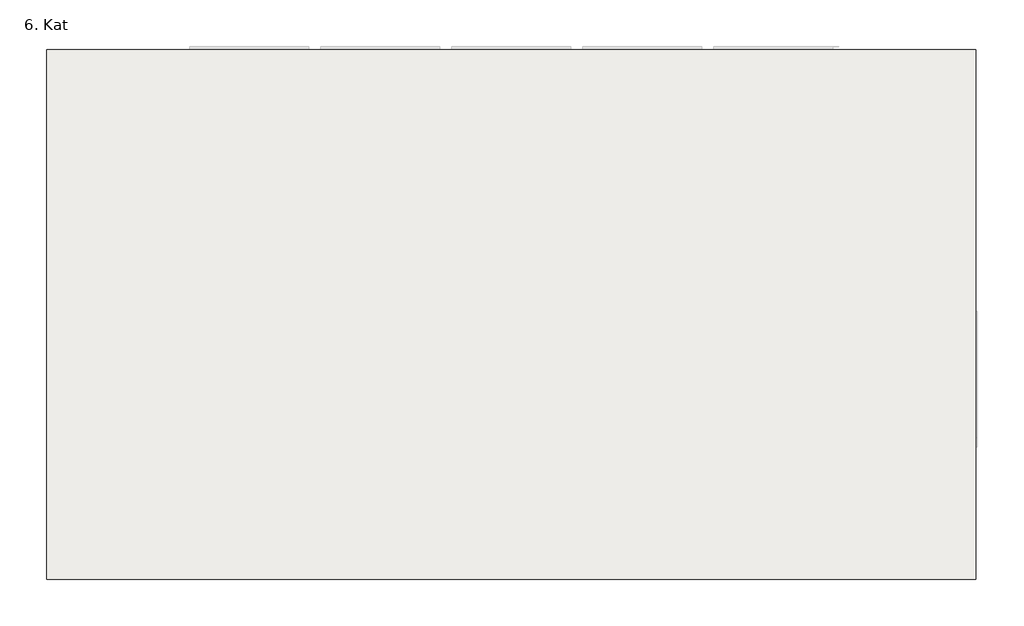
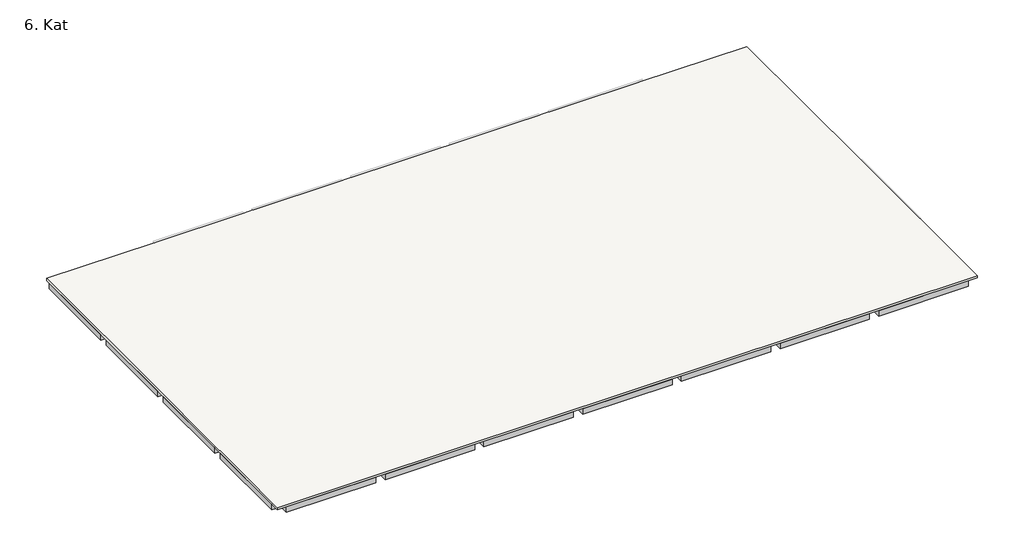
# One storey, part 1 of 2: 41 beams, 1 slab.
"""IFC4 building model written with IfcOpenShell, lengths in millimetres."""

from ifc_helpers import new_model, si_unit, frame, origin, place, context, project, spatial, polyline, outline, extrude, faceted_brep, element, save

model = new_model("IFC4")

# Units and contexts
model_context = context("Model", 3, world=origin())
ifc_project = project(units=[si_unit("LENGTHUNIT", "METRE", prefix="MILLI")], contexts=[model_context])

# Site, building, storey
site = spatial("IfcSite", under=ifc_project)
building = spatial("IfcBuilding", under=site)
storey = spatial("IfcBuildingStorey", under=building, Name="6. Kat", Elevation=31100.0)

# Beams
placement = place(None, origin())
element("IfcBeam", 1, ObjectType="M_Concrete-Rectangular Beam : 60x70cm kiriş", at=placement, inside=storey, context=model_context, shape_type="SweptSolid", body=[
    extrude(outline(polyline([(199.9996111, 8099.9999582), (199.9996111, 399.9999408), (-400.0003889, 399.9999408), (-400.0003889, 8099.9999582), (199.9996111, 8099.9999582)])), frame((0.0, 0.0, 30400.0), z_axis=(0.0, 0.0, 1.0), x_axis=(1.0, 0.0, 0.0)), (0.0, 0.0, 1.0), 500.0),
])
element("IfcBeam", 2, ObjectType="M_Concrete-Rectangular Beam : 60x70cm kiriş", at=placement, inside=storey, context=model_context, shape_type="SweptSolid", body=[
    extrude(outline(polyline([(199.9996411, 16599.9999423), (199.9996411, 8899.9999251), (-400.0003589, 8899.9999251), (-400.0003589, 16599.9999423), (199.9996411, 16599.9999423)])), frame((0.0, 0.0, 30400.0), z_axis=(0.0, 0.0, 1.0), x_axis=(1.0, 0.0, 0.0)), (0.0, 0.0, 1.0), 500.0),
])
element("IfcBeam", 3, ObjectType="M_Concrete-Rectangular Beam : 60x70cm kiriş", at=placement, inside=storey, context=model_context, shape_type="Brep", body=[
    faceted_brep([(199.9994072, 17399.9999423, 30400.0), (199.9994072, 23399.9999249, 30400.0), (199.9994072, 23899.9999249, 30400.0), (199.9994072, 25099.999926, 30400.0), (199.9994072, 25099.999926, 30900.0), (199.9994072, 23899.9999249, 30900.0), (199.9994072, 23399.9999249, 30900.0), (199.9994072, 17399.9999423, 30900.0), (-400.0005928, 17399.9999423, 30400.0), (-400.0005928, 25099.999926, 30400.0), (-400.0005928, 17399.9999423, 30900.0), (-400.0005928, 25099.999926, 30900.0)], [[[0, 1, 2, 3, 4, 5, 6, 7]], [[3, 2, 1, 0, 8, 9]], [[9, 8, 10, 11]], [[7, 6, 5, 4, 11, 10]], [[8, 0, 7, 10]], [[3, 9, 11, 4]]]),
])
element("IfcBeam", 4, ObjectType="M_Concrete-Rectangular Beam : 60x70cm kiriş", at=placement, inside=storey, context=model_context, shape_type="SweptSolid", body=[
    extrude(outline(polyline([(199.9994681, 25899.9999188), (-400.0005319, 25899.9999188), (-400.0005319, 33600.0004302), (199.9994681, 33600.0004302), (199.9994681, 25899.9999188)])), frame((0.0, 0.0, 30400.0), z_axis=(0.0, 0.0, 1.0), x_axis=(1.0, 0.0, 0.0)), (0.0, 0.0, 1.0), 500.0),
])
element("IfcBeam", 5, ObjectType="M_Concrete-Rectangular Beam : 60x70cm kiriş", at=placement, inside=storey, context=model_context, shape_type="SweptSolid", body=[
    extrude(outline(polyline([(8099.9996095, -400.0004808), (399.9996111, -400.0004808), (399.9996111, 199.9995192), (8099.9996095, 199.9995192), (8099.9996095, -400.0004808)])), frame((0.0, 0.0, 30400.0), z_axis=(0.0, 0.0, 1.0), x_axis=(1.0, 0.0, 0.0)), (0.0, 0.0, 1.0), 500.0),
])
element("IfcBeam", 6, ObjectType="M_Concrete-Rectangular Beam : 60x70cm kiriş", at=placement, inside=storey, context=model_context, shape_type="SweptSolid", body=[
    extrude(outline(polyline([(16599.9996095, -400.0000423), (8899.9996095, -400.0000423), (8899.9996095, 199.9999577), (16599.9996095, 199.9999577), (16599.9996095, -400.0000423)])), frame((0.0, 0.0, 30400.0), z_axis=(0.0, 0.0, 1.0), x_axis=(1.0, 0.0, 0.0)), (0.0, 0.0, 1.0), 500.0),
])
element("IfcBeam", 7, ObjectType="M_Concrete-Rectangular Beam : 60x70cm kiriş", at=placement, inside=storey, context=model_context, shape_type="SweptSolid", body=[
    extrude(outline(polyline([(25099.9996096, -399.9996163), (17399.9993907, -399.9996163), (17399.9993907, 200.0003837), (25099.9996096, 200.0003837), (25099.9996096, -399.9996163)])), frame((0.0, 0.0, 30400.0), z_axis=(0.0, 0.0, 1.0), x_axis=(1.0, 0.0, 0.0)), (0.0, 0.0, 1.0), 500.0),
])
element("IfcBeam", 8, ObjectType="M_Concrete-Rectangular Beam : 60x70cm kiriş", at=placement, inside=storey, context=model_context, shape_type="SweptSolid", body=[
    extrude(outline(polyline([(8899.9996095, 8100.0003637), (8899.9996095, 399.9999384), (8299.9996095, 399.9999384), (8299.9996095, 8100.0003637), (8899.9996095, 8100.0003637)])), frame((0.0, 0.0, 30400.0), z_axis=(0.0, 0.0, 1.0), x_axis=(1.0, 0.0, 0.0)), (0.0, 0.0, 1.0), 500.0),
])
element("IfcBeam", 9, ObjectType="M_Concrete-Rectangular Beam : 60x70cm kiriş", at=placement, inside=storey, context=model_context, shape_type="Brep", body=[
    faceted_brep([(8899.9996095, 8900.0003637, 30400.0), (8899.9996095, 13300.0003638, 30400.0), (8899.9996095, 13700.0003638, 30400.0), (8899.9996095, 16599.9999418, 30400.0), (8899.9996095, 16599.9999418, 30900.0), (8899.9996095, 13700.0003638, 30900.0), (8899.9996095, 13300.0003638, 30900.0), (8899.9996095, 8900.0003637, 30900.0), (8299.9996095, 8900.0003637, 30400.0), (8299.9996095, 16599.9999418, 30400.0), (8299.9996095, 8900.0003637, 30900.0), (8299.9996095, 16599.9999418, 30900.0)], [[[0, 1, 2, 3, 4, 5, 6, 7]], [[3, 2, 1, 0, 8, 9]], [[9, 8, 10, 11]], [[7, 6, 5, 4, 11, 10]], [[8, 0, 7, 10]], [[3, 9, 11, 4]]]),
])
element("IfcBeam", 10, ObjectType="M_Concrete-Rectangular Beam : 60x70cm kiriş", at=placement, inside=storey, context=model_context, shape_type="Brep", body=[
    faceted_brep([(8899.9996735, 25100.0003646, 30400.0), (8899.9996735, 25100.0003646, 30900.0), (8899.9996735, 17400.0009197, 30900.0), (8899.9996735, 17400.0009197, 30400.0), (8299.9996735, 25100.0003646, 30400.0), (8299.9996735, 17400.0009197, 30400.0), (8299.9996735, 18150.0006424, 30400.0), (8299.9996735, 18550.0006424, 30400.0), (8299.9996735, 23399.9999249, 30400.0), (8299.9996735, 23899.9999249, 30400.0), (8299.9996735, 25100.0003646, 30900.0), (8299.9996735, 17400.0009197, 30900.0), (8299.9996735, 18150.0006424, 30900.0), (8299.9996735, 18550.0006424, 30900.0), (8299.9996735, 23399.9999249, 30900.0), (8299.9996735, 23899.9999249, 30900.0)], [[[0, 1, 2, 3]], [[4, 0, 3, 5, 6, 7, 8, 9]], [[10, 4, 9, 8, 7, 6, 5, 11, 12, 13, 14, 15]], [[1, 10, 15, 14, 13, 12, 11, 2]], [[0, 4, 10, 1]], [[3, 2, 11, 5]]]),
])
element("IfcBeam", 11, ObjectType="M_Concrete-Rectangular Beam : 60x70cm kiriş", at=placement, inside=storey, context=model_context, shape_type="SweptSolid", body=[
    extrude(outline(polyline([(8899.9993907, 25899.9999188), (8299.9993907, 25899.9999188), (8299.9993907, 33600.0004302), (8899.9993907, 33600.0004302), (8899.9993907, 25899.9999188)])), frame((0.0, 0.0, 30400.0), z_axis=(0.0, 0.0, 1.0), x_axis=(1.0, 0.0, 0.0)), (0.0, 0.0, 1.0), 500.0),
])
element("IfcBeam", 12, ObjectType="M_Concrete-Rectangular Beam : 60x70cm kiriş", at=placement, inside=storey, context=model_context, shape_type="SweptSolid", body=[
    extrude(outline(polyline([(8099.9997323, 25299.999992), (399.9997323, 25299.999992), (399.9997323, 25899.999992), (8099.9997323, 25899.999992), (8099.9997323, 25299.999992)])), frame((0.0, 0.0, 30400.0), z_axis=(0.0, 0.0, 1.0), x_axis=(1.0, 0.0, 0.0)), (0.0, 0.0, 1.0), 500.0),
])
element("IfcBeam", 13, ObjectType="M_Concrete-Rectangular Beam : 50x70cm kiriş", at=placement, inside=storey, context=model_context, shape_type="SweptSolid", body=[
    extrude(outline(polyline([(199.9994072, 23399.9999249), (199.9994072, 23899.9999249), (8299.9996735, 23899.9999249), (8299.9996735, 23399.9999249), (199.9994072, 23399.9999249)])), frame((0.0, 0.0, 30400.0), z_axis=(0.0, 0.0, 1.0), x_axis=(1.0, 0.0, 0.0)), (0.0, 0.0, 1.0), 500.0),
])
element("IfcBeam", 14, ObjectType="M_Concrete-Rectangular Beam : 60x70cm kiriş", at=placement, inside=storey, context=model_context, shape_type="SweptSolid", body=[
    extrude(outline(polyline([(8099.9997451, 8200.0009197), (399.9996411, 8200.0009197), (399.9996411, 8800.0009197), (8099.9997451, 8800.0009197), (8099.9997451, 8200.0009197)])), frame((0.0, 0.0, 30400.0), z_axis=(0.0, 0.0, 1.0), x_axis=(1.0, 0.0, 0.0)), (0.0, 0.0, 1.0), 500.0),
])
element("IfcBeam", 15, ObjectType="M_Concrete-Rectangular Beam : 60x70cm kiriş", at=placement, inside=storey, context=model_context, shape_type="SweptSolid", body=[
    extrude(outline(polyline([(8099.9993907, 16800.0003638), (400.0000836, 16800.0003638), (400.0000836, 17400.0003638), (8099.9993907, 17400.0003638), (8099.9993907, 16800.0003638)])), frame((0.0, 0.0, 30400.0), z_axis=(0.0, 0.0, 1.0), x_axis=(1.0, 0.0, 0.0)), (0.0, 0.0, 1.0), 500.0),
])
element("IfcBeam", 16, ObjectType="M_Concrete-Rectangular Beam : 40x70cm kiriş 2", at=placement, inside=storey, context=model_context, shape_type="SweptSolid", body=[
    extrude(outline(polyline([(204.0222331, 18150.0006424), (204.0222331, 18550.0006424), (8299.9996735, 18550.0006424), (8299.9996735, 18150.0006424), (204.0222331, 18150.0006424)])), frame((0.0, 0.0, 30400.0), z_axis=(0.0, 0.0, 1.0), x_axis=(1.0, 0.0, 0.0)), (0.0, 0.0, 1.0), 500.0),
])
element("IfcBeam", 17, ObjectType="M_Concrete-Rectangular Beam : 60x70cm kiriş", at=placement, inside=storey, context=model_context, shape_type="SweptSolid", body=[
    extrude(outline(polyline([(8899.9993907, 25299.9999925), (8899.9993907, 25899.9999925), (12300.0064017, 25899.9999925), (12300.0064017, 25299.9999925), (8899.9993907, 25299.9999925)])), frame((0.0, 0.0, 30400.0), z_axis=(0.0, 0.0, 1.0), x_axis=(1.0, 0.0, 0.0)), (0.0, 0.0, 1.0), 500.0),
])
element("IfcBeam", 18, ObjectType="M_Concrete-Rectangular Beam : 60x70cm kiriş", at=placement, inside=storey, context=model_context, shape_type="Brep", body=[
    faceted_brep([(8899.9993907, 16800.0003643, 30900.0), (8899.9993907, 16800.0003643, 30400.0), (12300.0064017, 16800.0003643, 30400.0), (12300.0064017, 16800.0003643, 30900.0), (8899.9996735, 17400.0003643, 30400.0), (12300.0064017, 17400.0003643, 30400.0), (8899.9996735, 17400.0003643, 30900.0), (12300.0064017, 17400.0003643, 30900.0)], [[[0, 1, 2, 3]], [[1, 4, 5, 2]], [[4, 6, 7, 5]], [[6, 4, 1, 0]], [[6, 0, 3, 7]], [[3, 2, 5, 7]]]),
])
element("IfcBeam", 19, ObjectType="M_Concrete-Rectangular Beam : 40x70cm kiriş 2", at=placement, inside=storey, context=model_context, shape_type="Brep", body=[
    faceted_brep([(12700.0064017, 17000.0003638, 30900.0), (12700.0064017, 17000.0003638, 30400.0), (14600.0010318, 17000.0003638, 30400.0), (14900.0010318, 17000.0003638, 30400.0), (16999.9995362, 17000.0003638, 30400.0), (16999.9995362, 17000.0003638, 30900.0), (14900.0010318, 17000.0003638, 30900.0), (14600.0010318, 17000.0003638, 30900.0), (12700.0064017, 17400.0003638, 30400.0), (16999.9995362, 17400.0003638, 30400.0), (12700.0064017, 17400.0003638, 30900.0), (16999.9995362, 17400.0003638, 30900.0)], [[[0, 1, 2, 3, 4, 5, 6, 7]], [[1, 8, 9, 4, 3, 2]], [[8, 10, 11, 9]], [[10, 0, 7, 6, 5, 11]], [[8, 1, 0, 10]], [[5, 4, 9, 11]]]),
])
element("IfcBeam", 20, ObjectType="M_Concrete-Rectangular Beam : 40x70cm kiriş 2", at=placement, inside=storey, context=model_context, shape_type="SweptSolid", body=[
    extrude(outline(polyline([(25099.999715, 17400.0003766), (25099.999715, 17000.0003766), (17399.9995362, 17000.0003766), (17399.9995362, 17400.0003766), (25099.999715, 17400.0003766)])), frame((0.0, 0.0, 30400.0), z_axis=(0.0, 0.0, 1.0), x_axis=(1.0, 0.0, 0.0)), (0.0, 0.0, 1.0), 500.0),
])
element("IfcBeam", 21, ObjectType="M_Concrete-Rectangular Beam : 40x70cm kiriş 2", at=placement, inside=storey, context=model_context, shape_type="Brep", body=[
    faceted_brep([(16599.9993867, 13700.0003638, 30400.0), (14900.0010318, 13700.0003638, 30400.0), (14600.0010318, 13700.0003638, 30400.0), (12700.0064017, 13700.0003638, 30400.0), (12300.0064017, 13700.0003638, 30400.0), (8899.9996095, 13700.0003638, 30400.0), (8899.9996095, 13700.0003638, 30900.0), (12300.0064017, 13700.0003638, 30900.0), (12700.0064017, 13700.0003638, 30900.0), (14600.0010318, 13700.0003638, 30900.0), (14900.0010318, 13700.0003638, 30900.0), (16599.9993867, 13700.0003638, 30900.0), (16599.9993867, 13300.0003638, 30400.0), (12700.0064017, 13300.0003638, 30400.0), (12300.0064017, 13300.0003638, 30400.0), (8899.9996095, 13300.0003638, 30400.0), (16599.9993867, 13300.0003638, 30900.0), (12700.0064017, 13300.0003638, 30900.0), (12300.0064017, 13300.0003638, 30900.0), (8899.9996095, 13300.0003638, 30900.0)], [[[0, 1, 2, 3, 4, 5, 6, 7, 8, 9, 10, 11]], [[5, 4, 3, 2, 1, 0, 12, 13, 14, 15]], [[15, 14, 13, 12, 16, 17, 18, 19]], [[5, 15, 19, 6]], [[11, 10, 9, 8, 7, 6, 19, 18, 17, 16]], [[12, 0, 11, 16]]]),
])
element("IfcBeam", 22, ObjectType="M_Concrete-Rectangular Beam : 40x70cm kiriş 2", at=placement, inside=storey, context=model_context, shape_type="SweptSolid", body=[
    extrude(outline(polyline([(12300.0064017, 16037.3003638), (12700.0064017, 16037.3003638), (12700.0064017, 13700.0003638), (12300.0064017, 13700.0003638), (12300.0064017, 16037.3003638)])), frame((0.0, 0.0, 30400.0), z_axis=(0.0, 0.0, 1.0), x_axis=(1.0, 0.0, 0.0)), (0.0, 0.0, 1.0), 500.0),
])
element("IfcBeam", 23, ObjectType="M_Concrete-Rectangular Beam : 40x70cm kiriş 2", at=placement, inside=storey, context=model_context, shape_type="SweptSolid", body=[
    extrude(outline(polyline([(16999.9995362, 16037.3003638), (17399.9995362, 16037.3003638), (17399.9995362, 14099.9451047), (16999.9995362, 14099.9451047), (16999.9995362, 16037.3003638)])), frame((0.0, 0.0, 30400.0), z_axis=(0.0, 0.0, 1.0), x_axis=(1.0, 0.0, 0.0)), (0.0, 0.0, 1.0), 500.0),
])
element("IfcBeam", 24, ObjectType="M_Concrete-Rectangular Beam : 30x70cm kiriş 3", at=placement, inside=storey, context=model_context, shape_type="Brep", body=[
    faceted_brep([(12700.0064017, 16350.0003638, 30400.0), (12700.0064017, 16350.0003638, 30900.0), (14600.0010318, 16350.0003638, 30900.0), (14900.0010318, 16350.0003638, 30900.0), (16999.9995362, 16350.0003638, 30900.0), (16999.9995362, 16350.0003638, 30400.0), (14900.0010318, 16350.0003638, 30400.0), (14600.0010318, 16350.0003638, 30400.0), (12700.0064017, 16050.0003638, 30400.0), (16999.9995362, 16050.0003638, 30400.0), (14900.0010318, 16050.0003638, 30400.0), (14600.0010318, 16050.0003638, 30400.0), (12700.0064017, 16050.0003638, 30900.0), (16999.9995362, 16050.0003638, 30900.0), (14900.0010318, 16050.0003638, 30900.0), (14600.0010318, 16050.0003638, 30900.0)], [[[0, 1, 2, 3, 4, 5, 6, 7]], [[8, 0, 7, 6, 5, 9, 10, 11]], [[12, 8, 11, 10, 9, 13, 14, 15]], [[1, 12, 15, 14, 13, 4, 3, 2]], [[1, 0, 8, 12]], [[5, 4, 13, 9]]]),
])
element("IfcBeam", 25, ObjectType="M_Concrete-Rectangular Beam : 30x70cm kiriş 3", at=placement, inside=storey, context=model_context, shape_type="SweptSolid", body=[
    extrude(outline(polyline([(14900.0010318, 13700.0003638), (14600.0010318, 13700.0003638), (14600.0010318, 16050.0003638), (14900.0010318, 16050.0003638), (14900.0010318, 13700.0003638)])), frame((0.0, 0.0, 30400.0), z_axis=(0.0, 0.0, 1.0), x_axis=(1.0, 0.0, 0.0)), (0.0, 0.0, 1.0), 500.0),
    extrude(outline(polyline([(14600.0010318, 17000.0003638), (14900.0010318, 17000.0003638), (14900.0010318, 16350.0003638), (14600.0010318, 16350.0003638), (14600.0010318, 17000.0003638)])), frame((0.0, 0.0, 30400.0), z_axis=(0.0, 0.0, 1.0), x_axis=(1.0, 0.0, 0.0)), (0.0, 0.0, 1.0), 500.0),
])
element("IfcBeam", 26, ObjectType="M_Concrete-Rectangular Beam : 60x70cm kiriş", at=placement, inside=storey, context=model_context, shape_type="Brep", body=[
    faceted_brep([(8899.9993907, 8200.0009197, 30400.0), (16599.9993907, 8200.0009197, 30400.0), (16599.9993907, 8200.0009197, 30900.0), (8899.9993907, 8200.0009197, 30900.0), (8899.9993907, 8800.0009197, 30400.0), (12300.0064017, 8800.0009197, 30400.0), (12700.0064017, 8800.0009197, 30400.0), (16599.9993907, 8800.0009197, 30400.0), (8899.9993907, 8800.0009197, 30900.0), (12300.0064017, 8800.0009197, 30900.0), (12700.0064017, 8800.0009197, 30900.0), (16599.9993907, 8800.0009197, 30900.0)], [[[0, 1, 2, 3]], [[1, 0, 4, 5, 6, 7]], [[7, 6, 5, 4, 8, 9, 10, 11]], [[3, 2, 11, 10, 9, 8]], [[4, 0, 3, 8]], [[1, 7, 11, 2]]]),
])
element("IfcBeam", 27, ObjectType="M_Concrete-Rectangular Beam : 60x70cm kiriş", at=placement, inside=storey, context=model_context, shape_type="SweptSolid", body=[
    extrude(outline(polyline([(17399.9997293, 8900.0009197), (16799.9997293, 8900.0009197), (16799.9997293, 13299.9451047), (17399.9997293, 13299.9451047), (17399.9997293, 8900.0009197)])), frame((0.0, 0.0, 30400.0), z_axis=(0.0, 0.0, 1.0), x_axis=(1.0, 0.0, 0.0)), (0.0, 0.0, 1.0), 500.0),
])
element("IfcBeam", 28, ObjectType="M_Concrete-Rectangular Beam : 60x70cm kiriş", at=placement, inside=storey, context=model_context, shape_type="SweptSolid", body=[
    extrude(outline(polyline([(16799.9997451, 400.0009197), (16799.9997451, 8099.9999409), (17399.9997451, 8099.9999409), (17399.9997451, 400.0009197), (16799.9997451, 400.0009197)])), frame((0.0, 0.0, 30400.0), z_axis=(0.0, 0.0, 1.0), x_axis=(1.0, 0.0, 0.0)), (0.0, 0.0, 1.0), 500.0),
])
element("IfcBeam", 29, ObjectType="M_Concrete-Rectangular Beam : 40x70cm kiriş 2", at=placement, inside=storey, context=model_context, shape_type="SweptSolid", body=[
    extrude(outline(polyline([(12300.0064017, 13300.0003638), (12700.0064017, 13300.0003638), (12700.0064017, 8800.0009197), (12300.0064017, 8800.0009197), (12300.0064017, 13300.0003638)])), frame((0.0, 0.0, 30400.0), z_axis=(0.0, 0.0, 1.0), x_axis=(1.0, 0.0, 0.0)), (0.0, 0.0, 1.0), 500.0),
])
element("IfcBeam", 30, ObjectType="M_Concrete-Rectangular Beam : 60x70cm kiriş", at=placement, inside=storey, context=model_context, shape_type="SweptSolid", body=[
    extrude(outline(polyline([(25299.9997233, 400.0009197), (25299.9997233, 8100.0009197), (25899.9997233, 8100.0009197), (25899.9997233, 400.0009197), (25299.9997233, 400.0009197)])), frame((0.0, 0.0, 30400.0), z_axis=(0.0, 0.0, 1.0), x_axis=(1.0, 0.0, 0.0)), (0.0, 0.0, 1.0), 500.0),
])
element("IfcBeam", 31, ObjectType="M_Concrete-Rectangular Beam : 60x70cm kiriş", at=placement, inside=storey, context=model_context, shape_type="SweptSolid", body=[
    extrude(outline(polyline([(25099.9993907, 8200.0009197), (17399.9993907, 8200.0009197), (17399.9993907, 8800.0009197), (25099.9993907, 8800.0009197), (25099.9993907, 8200.0009197)])), frame((0.0, 0.0, 30400.0), z_axis=(0.0, 0.0, 1.0), x_axis=(1.0, 0.0, 0.0)), (0.0, 0.0, 1.0), 500.0),
])
element("IfcBeam", 32, ObjectType="M_Concrete-Rectangular Beam : 60x70cm kiriş", at=placement, inside=storey, context=model_context, shape_type="SweptSolid", body=[
    extrude(outline(polyline([(25899.9997233, 8900.0009197), (25299.9997233, 8900.0009197), (25299.9997233, 13300.0003995), (25899.9997233, 13300.0003995), (25899.9997233, 8900.0009197)])), frame((0.0, 0.0, 30400.0), z_axis=(0.0, 0.0, 1.0), x_axis=(1.0, 0.0, 0.0)), (0.0, 0.0, 1.0), 500.0),
])
element("IfcBeam", 33, ObjectType="M_Concrete-Rectangular Beam : 40x70cm kiriş 2", at=placement, inside=storey, context=model_context, shape_type="Brep", body=[
    faceted_brep([(25099.9997415, 13700.0003995, 30900.0), (25099.9997415, 13700.0003995, 30400.0), (17399.9993907, 13700.0003995, 30400.0), (17399.9993907, 13700.0003995, 30900.0), (17399.9997293, 13300.0003995, 30400.0), (25099.9997415, 13300.0003995, 30400.0), (17399.9997293, 13300.0003995, 30900.0), (25099.9997415, 13300.0003995, 30900.0)], [[[0, 1, 2, 3]], [[4, 2, 1, 5]], [[6, 4, 5, 7]], [[4, 6, 3, 2]], [[3, 6, 7, 0]], [[5, 1, 0, 7]]]),
])
element("IfcBeam", 34, ObjectType="M_Concrete-Rectangular Beam : 60x70cm kiriş", at=placement, inside=storey, context=model_context, shape_type="SweptSolid", body=[
    extrude(outline(polyline([(25299.9997233, 14100.0003995), (25299.9997233, 16600.0009197), (25899.9997233, 16600.0009197), (25899.9997233, 14100.0003995), (25299.9997233, 14100.0003995)])), frame((0.0, 0.0, 30400.0), z_axis=(0.0, 0.0, 1.0), x_axis=(1.0, 0.0, 0.0)), (0.0, 0.0, 1.0), 500.0),
])
element("IfcBeam", 35, ObjectType="M_Concrete-Rectangular Beam : 40x70cm kiriş 2", at=placement, inside=storey, context=model_context, shape_type="Brep", body=[
    faceted_brep([(33599.9993907, 17000.0007711, 30400.0), (33599.9993907, 17000.0007711, 30900.0), (25899.9993907, 17000.0007711, 30900.0), (25899.9993907, 17000.0007711, 30400.0), (25899.999682, 17400.0007711, 30400.0), (33599.9994953, 17400.0007711, 30400.0), (25899.999682, 17400.0007711, 30900.0), (33599.9994953, 17400.0007711, 30900.0)], [[[0, 1, 2, 3]], [[3, 4, 5, 0]], [[4, 6, 7, 5]], [[3, 2, 6, 4]], [[5, 7, 1, 0]], [[7, 6, 2, 1]]]),
])
element("IfcBeam", 36, ObjectType="M_Concrete-Rectangular Beam : 40x70cm kiriş 2", at=placement, inside=storey, context=model_context, shape_type="Brep", body=[
    faceted_brep([(25899.9997233, 13300.0003995, 30900.0), (25899.9997233, 13300.0003995, 30400.0), (33599.9993907, 13300.0003995, 30400.0), (33599.9993907, 13300.0003995, 30900.0), (25899.9993907, 13700.0003995, 30400.0), (33599.9993907, 13700.0003995, 30400.0), (33599.9993907, 13700.0003995, 30900.0), (25899.9993907, 13700.0003995, 30900.0)], [[[0, 1, 2, 3]], [[1, 4, 5, 2]], [[6, 5, 4, 7]], [[1, 0, 7, 4]], [[7, 0, 3, 6]], [[3, 2, 5, 6]]]),
])
element("IfcBeam", 37, ObjectType="M_Concrete-Rectangular Beam : 60x70cm kiriş", at=placement, inside=storey, context=model_context, shape_type="Brep", body=[
    faceted_brep([(25899.9993907, 8200.0009197, 30900.0), (25899.9993907, 8200.0009197, 30400.0), (33599.9993907, 8200.0009197, 30400.0), (33599.9993907, 8200.0009197, 30900.0), (33599.9994953, 8800.0009197, 30400.0), (25899.9993907, 8800.0009197, 30400.0), (33599.9994953, 8800.0009197, 30900.0), (25899.9993907, 8800.0009197, 30900.0)], [[[0, 1, 2, 3]], [[4, 2, 1, 5]], [[6, 4, 5, 7]], [[4, 6, 3, 2]], [[3, 6, 7, 0]], [[1, 0, 7, 5]]]),
])
element("IfcBeam", 38, ObjectType="M_Concrete-Rectangular Beam : 60x70cm kiriş", at=placement, inside=storey, context=model_context, shape_type="Brep", body=[
    faceted_brep([(34399.9993907, -399.9996882, 30900.0), (34399.9993907, -399.9996882, 30400.0), (42099.9993899, -399.9996882, 30400.0), (42099.9993899, -399.9996882, 30900.0), (42099.999723, 200.0003118, 30400.0), (34399.9993907, 200.0003118, 30400.0), (42099.999723, 200.0003118, 30900.0), (34399.9993907, 200.0003118, 30900.0)], [[[0, 1, 2, 3]], [[4, 2, 1, 5]], [[6, 4, 5, 7]], [[4, 6, 3, 2]], [[3, 6, 7, 0]], [[1, 0, 7, 5]]]),
])
element("IfcBeam", 39, ObjectType="M_Concrete-Rectangular Beam : 60x70cm kiriş", at=placement, inside=storey, context=model_context, shape_type="SweptSolid", body=[
    extrude(outline(polyline([(25899.9993907, -399.9996882), (25899.9993907, 200.0003118), (33599.9993907, 200.0003118), (33599.9993907, -399.9996882), (25899.9993907, -399.9996882)])), frame((0.0, 0.0, 30400.0), z_axis=(0.0, 0.0, 1.0), x_axis=(1.0, 0.0, 0.0)), (0.0, 0.0, 1.0), 500.0),
])
element("IfcBeam", 40, ObjectType="M_Concrete-Rectangular Beam : 60x70cm kiriş", at=placement, inside=storey, context=model_context, shape_type="Brep", body=[
    faceted_brep([(42899.9997771, -399.9996882, 30900.0), (42899.9997771, -399.9996882, 30400.0), (50599.9993899, -399.9996882, 30400.0), (50599.9993899, -399.9996882, 30900.0), (50599.999723, 200.0003118, 30400.0), (42899.9997771, 200.0003118, 30400.0), (50599.999723, 200.0003118, 30900.0), (42899.9997771, 200.0003118, 30900.0)], [[[0, 1, 2, 3]], [[4, 2, 1, 5]], [[6, 4, 5, 7]], [[4, 6, 3, 2]], [[3, 6, 7, 0]], [[5, 1, 0, 7]]]),
])
element("IfcBeam", 41, ObjectType="M_Concrete-Rectangular Beam : 60x70cm kiriş", at=placement, inside=storey, context=model_context, shape_type="SweptSolid", body=[
    extrude(outline(polyline([(59099.9997769, -399.9996882), (51399.9997769, -399.9996882), (51399.9997769, 200.0003118), (59099.9997769, 200.0003118), (59099.9997769, -399.9996882)])), frame((0.0, 0.0, 30400.0), z_axis=(0.0, 0.0, 1.0), x_axis=(1.0, 0.0, 0.0)), (0.0, 0.0, 1.0), 500.0),
])

# Slab
element("IfcSlab", 42, ObjectType="20 cm döşeme", at=placement, inside=storey, context=model_context, shape_type="Brep", body=[
    faceted_brep([(59899.9997758, 34000.0004302, 30900.0), (59899.9997758, 16600.0009197, 30900.0), (59899.9997758, 8900.0009197, 30900.0), (59899.9997758, -399.9995292, 30900.0), (-400.0005319, -399.9995292, 30900.0), (-400.0005319, 25899.9999188, 30900.0), (-400.0005319, 33600.0004302, 30900.0), (-400.0005319, 34000.0004302, 30900.0), (8899.9993907, 34000.0004302, 30900.0), (16599.9993907, 34000.0004302, 30900.0), (17399.9993907, 34000.0004302, 30900.0), (25099.9993907, 34000.0004302, 30900.0), (25899.9993907, 34000.0004302, 30900.0), (33599.9993907, 34000.0004302, 30900.0), (34399.9993907, 34000.0004302, 30900.0), (42099.9993899, 34000.0004302, 30900.0), (42899.999681, 34000.0004302, 30900.0), (50599.9994944, 34000.0004302, 30900.0), (59899.9997758, 34000.0004302, 31100.0), (50599.9994944, 34000.0004302, 31100.0), (42899.999681, 34000.0004302, 31100.0), (42099.9993899, 34000.0004302, 31100.0), (34399.9993907, 34000.0004302, 31100.0), (33599.9993907, 34000.0004302, 31100.0), (25899.9993907, 34000.0004302, 31100.0), (25099.9993907, 34000.0004302, 31100.0), (17399.9993907, 34000.0004302, 31100.0), (16599.9993907, 34000.0004302, 31100.0), (8899.9995273, 34000.0004302, 31100.0), (-400.0005319, 34000.0004302, 31100.0), (-400.0005319, -399.9995292, 31100.0), (59899.9997758, -399.9995292, 31100.0), (59899.9997758, 8200.0009197, 31100.0), (59899.9997758, 8800.0009197, 31100.0), (59899.9997758, 17000.0009197, 31100.0)], [[[0, 1, 2, 3, 4, 5, 6, 7, 8, 9, 10, 11, 12, 13, 14, 15, 16, 17]], [[18, 19, 20, 21, 22, 23, 24, 25, 26, 27, 28, 29, 30, 31, 32, 33, 34]], [[3, 2, 1, 0, 18, 34, 33, 32, 31]], [[4, 3, 31, 30]], [[7, 6, 5, 4, 30, 29]], [[0, 17, 16, 15, 14, 13, 12, 11, 10, 9, 8, 7, 29, 28, 27, 26, 25, 24, 23, 22, 21, 20, 19, 18]]]),
])

save(model, "model.ifc")

# Revit data of these elements
# Type "M_Concrete-Rectangular Beam : 60x70cm kiriş"
#   Length [instance default] = 152.4 cm
#   b = 60 cm
#   h = 70 cm
#   Structural Material [instance default] = Concrete, Cast-in-Place gray
#   Assembly Code = ""
# Type "M_Concrete-Rectangular Beam : 50x70cm kiriş"
#   Length [instance default] = 152.4 cm
#   b = 50 cm
#   h = 70 cm
#   Structural Material [instance default] = Concrete, Cast-in-Place gray
#   Assembly Code = ""
# Type "M_Concrete-Rectangular Beam : 40x70cm kiriş 2"
#   Length [instance default] = 152.4 cm
#   b = 40 cm
#   h = 70 cm
#   Structural Material [instance default] = Concrete, Cast-in-Place gray
#   Assembly Code = ""
# Type "M_Concrete-Rectangular Beam : 30x70cm kiriş 3"
#   Length [instance default] = 152.4 cm
#   b = 30 cm
#   h = 70 cm
#   Structural Material [instance default] = Concrete, Cast-in-Place gray
#   Assembly Code = ""
# Type "20 cm döşeme"
#   Function = 0
#   Layers, outside or top first: 20 cm no material (function 1)
# Elements 1, 2, 3, 4, 5, 6, 7, 8, 9, 10, 11, 12, 14, 15, 17, 18, 26, 27, 28, 30, 31, 32, 34, 37, 38, 39, 40, 41 (IfcBeam, "M_Concrete-Rectangular Beam : 60x70cm kiriş")
#   Comments = ""
#   Structural Material = Concrete, Cast-in-Place gray
#   Phase Created = New Construction
#   Materials on its faces: "Concrete, Cast-in-Place gray"
# Element 13 (IfcBeam, "M_Concrete-Rectangular Beam : 50x70cm kiriş")
#   Comments = ""
#   Structural Material = Concrete, Cast-in-Place gray
#   Phase Created = New Construction
#   Materials on its faces: "Concrete, Cast-in-Place gray"
# Elements 16, 19, 20, 21, 22, 23, 29, 33, 35, 36 (IfcBeam, "M_Concrete-Rectangular Beam : 40x70cm kiriş 2")
#   Comments = ""
#   Structural Material = Concrete, Cast-in-Place gray
#   Phase Created = New Construction
#   Materials on its faces: "Concrete, Cast-in-Place gray"
# Elements 24, 25 (IfcBeam, "M_Concrete-Rectangular Beam : 30x70cm kiriş 3")
#   Comments = ""
#   Structural Material = Concrete, Cast-in-Place gray
#   Phase Created = New Construction
#   Materials on its faces: "Concrete, Cast-in-Place gray"
# Element 42 (IfcSlab, "20 cm döşeme")
#   Height Offset From Level = 0 cm
#   built-in parameter 1001954 = 1
#   Phase Created = New Construction
#   Materials on its faces: "Default Floor"
# Materials
#   "Concrete, Cast-in-Place gray": class "Concrete", colour RGB 192 192 192, transparency 0, Description = "Cast-in-place concrete", Cost = 0
#   "Default Floor": class "Miscellaneous", colour RGB 127 127 127, transparency 0
